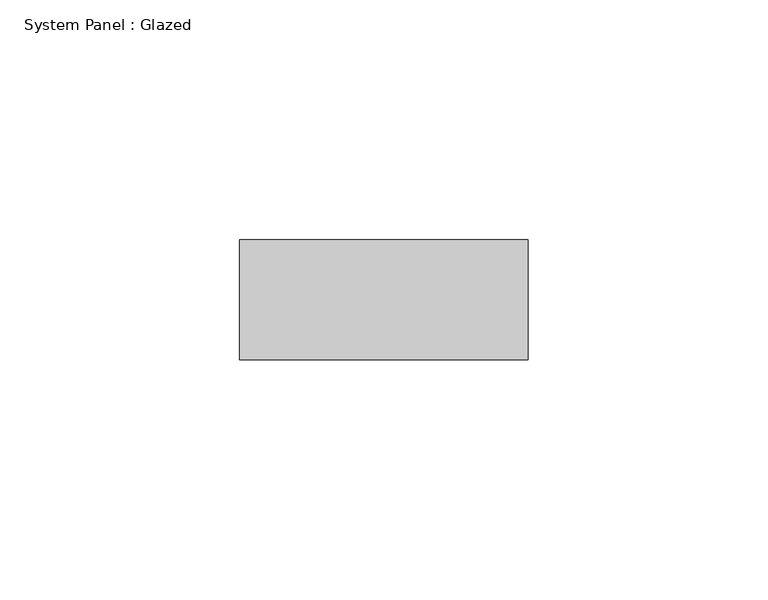
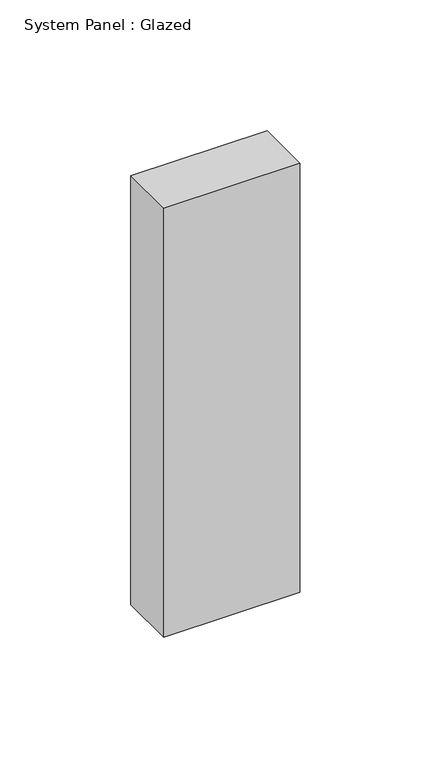
"""IFC4 building model written with IfcOpenShell, lengths in millimetres: plate geometry, System Panel : Glazed."""

from ifc_helpers import new_model, si_unit, origin, origin_with_axes, place, context, project, spatial, polyline, outline, extrude, source, transform, mapped, element, save


def system_panel_glazed_944c5575(model_context):
    return source(origin(), model_context, "Body", "SweptSolid", [
        extrude(outline(polyline([(30.0531077, 24.5), (-30.0531077, 24.5), (-30.0531077, 49.5), (30.0531077, 49.5), (30.0531077, 24.5)])), origin_with_axes(), (0.0, 0.0, 1.0), 200.0),
    ])


if __name__ == "__main__":
    model = new_model("IFC4")
    model_context = context("Model", 3, world=origin())
    ifc_project = project(units=[si_unit("LENGTHUNIT", "METRE", prefix="MILLI")], contexts=[model_context])
    site = spatial("IfcSite", under=ifc_project)
    building = spatial("IfcBuilding", under=site)
    placement = place(None, origin())
    system_panel_glazed_shape = system_panel_glazed_944c5575(model_context)
    element("IfcPlate", 1, ObjectType="System Panel : Glazed", at=placement, inside=building, context=model_context, shape_type="MappedRepresentation", body=[
        mapped(system_panel_glazed_shape, transform((0.0, 0.0, 0.0), x_axis=(1.0, 0.0, 0.0), y_axis=(0.0, 1.0, 0.0), z_axis=(0.0, 0.0, 1.0))),
    ])
    save(model, "model.ifc")

# Revit data of these elements
# Element 1 (IfcPlate, "System Panel : Glazed")
#   Materials on its faces: "Glass"
# Materials
#   "Glass": class "Glass", colour RGB 218 227 224, transparency 0.85, Description = "Soda Lime Glass", Cost = 0
